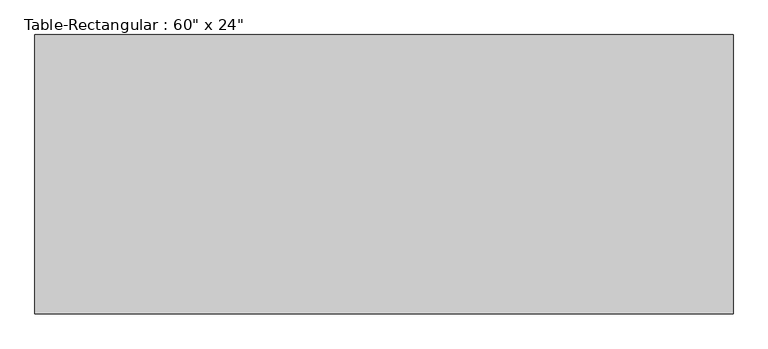
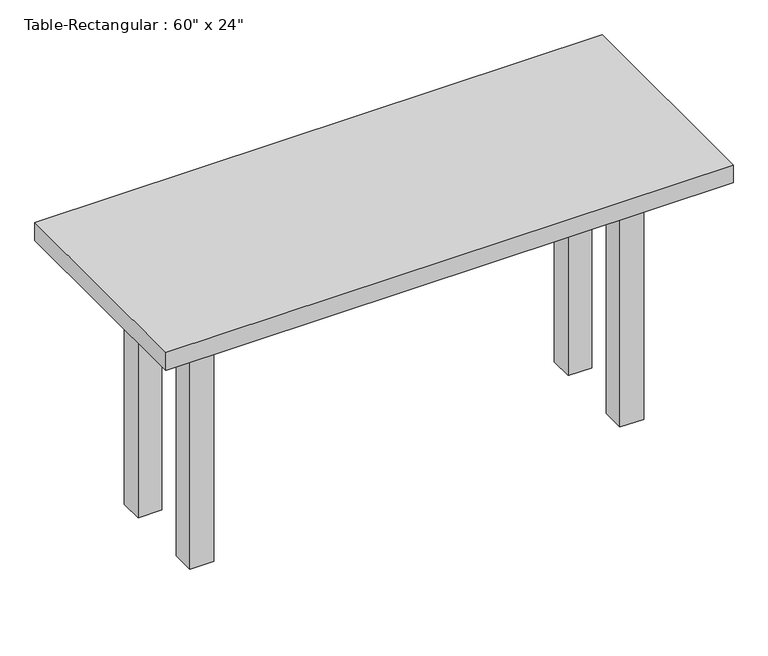
"""IFC4 building model written with IfcOpenShell, lengths in millimetres: furniture geometry."""

from ifc_helpers import new_model, si_unit, frame, origin, origin_with_axes, place, context, project, spatial, polyline, outline, extrude, source, transform, mapped, element, save


def furniture_b34bcf6c(model_context):
    return source(origin(), model_context, "Body", "SweptSolid", [
        extrude(outline(polyline([(546.1, -114.3), (-546.1, -114.3), (-546.1, -88.9), (546.1, -88.9), (546.1, -114.3)])), frame((0.0, 0.0, 609.6), z_axis=(0.0, 0.0, 1.0), x_axis=(1.0, 0.0, 0.0)), (0.0, 0.0, 1.0), 101.6),
        extrude(outline(polyline([(546.1, 114.3), (546.1, 88.9), (-546.1, 88.9), (-546.1, 114.3), (546.1, 114.3)])), frame((0.0, 0.0, 609.6), z_axis=(0.0, 0.0, 1.0), x_axis=(1.0, 0.0, 0.0)), (0.0, 0.0, 1.0), 101.6),
        extrude(outline(polyline([(-558.8, 88.9), (-558.8, -88.9), (-584.2, -88.9), (-584.2, 88.9), (-558.8, 88.9)])), frame((0.0, 0.0, 609.6), z_axis=(0.0, 0.0, 1.0), x_axis=(1.0, 0.0, 0.0)), (0.0, 0.0, 1.0), 101.6),
        extrude(outline(polyline([(558.8, 88.9), (584.2, 88.9), (584.2, -88.9), (558.8, -88.9), (558.8, 88.9)])), frame((0.0, 0.0, 609.6), z_axis=(0.0, 0.0, 1.0), x_axis=(1.0, 0.0, 0.0)), (0.0, 0.0, 1.0), 101.6),
        extrude(outline(polyline([(762.0, -304.8), (-762.0, -304.8), (-762.0, 304.8), (762.0, 304.8), (762.0, -304.8)])), frame((0.0, 0.0, 711.2), z_axis=(0.0, 0.0, 1.0), x_axis=(1.0, 0.0, 0.0)), (0.0, 0.0, 1.0), 50.8),
        extrude(outline(polyline([(-546.1, -152.4), (-609.6, -152.4), (-609.6, -88.9), (-546.1, -88.9), (-546.1, -152.4)])), origin_with_axes(), (0.0, 0.0, 1.0), 711.2),
        extrude(outline(polyline([(546.1, -152.4), (546.1, -88.9), (609.6, -88.9), (609.6, -152.4), (546.1, -152.4)])), origin_with_axes(), (0.0, 0.0, 1.0), 711.2),
        extrude(outline(polyline([(-546.1, 152.4), (-546.1, 88.9), (-609.6, 88.9), (-609.6, 152.4), (-546.1, 152.4)])), origin_with_axes(), (0.0, 0.0, 1.0), 711.2),
        extrude(outline(polyline([(546.1, 152.4), (609.6, 152.4), (609.6, 88.9), (546.1, 88.9), (546.1, 152.4)])), origin_with_axes(), (0.0, 0.0, 1.0), 711.2),
    ])


if __name__ == "__main__":
    model = new_model("IFC4")
    model_context = context("Model", 3, world=origin())
    ifc_project = project(units=[si_unit("LENGTHUNIT", "METRE", prefix="MILLI")], contexts=[model_context])
    site = spatial("IfcSite", under=ifc_project)
    building = spatial("IfcBuilding", under=site)
    placement = place(None, origin())
    furniture_shape = furniture_b34bcf6c(model_context)
    element("IfcFurniture", 1, ObjectType="Table-Rectangular : 60\" x 24\"", at=placement, inside=building, context=model_context, shape_type="MappedRepresentation", body=[
        mapped(furniture_shape, transform((0.0, 0.0, 0.0), x_axis=(1.0, 0.0, 0.0), y_axis=(0.0, 1.0, 0.0), z_axis=(0.0, 0.0, 1.0))),
    ])
    save(model, "model.ifc")

# Revit data of these elements
# Type "Table-Rectangular : 60\" x 24\""
#   Model = "Desk"
#   Manufacturer = "Acme Funriture"
#   Assembly Code = "E2020200"
#   Height = 2' - 6"
#   Length = 5' - 0"
#   Width = 2' - 0"
#   Base Material = Birch
#   Top Material = Laminate, Blue, Matte
#   Default Elevation = 0
# Element 1 (IfcFurniture, "Table-Rectangular : 60\" x 24\"")
#   Materials on its faces: "Birch", "Laminate, Blue, Matte"
# Materials
#   "Birch": class "Wood", colour RGB 172 132 95, transparency 0, Description = "Betula Alleghaniensis", Cost = 0
#   "Laminate, Blue, Matte": class "Plastic", colour RGB 85 101 155, transparency 0, Description = "Plastic Laminate - Blue, Matte", Cost = 0
